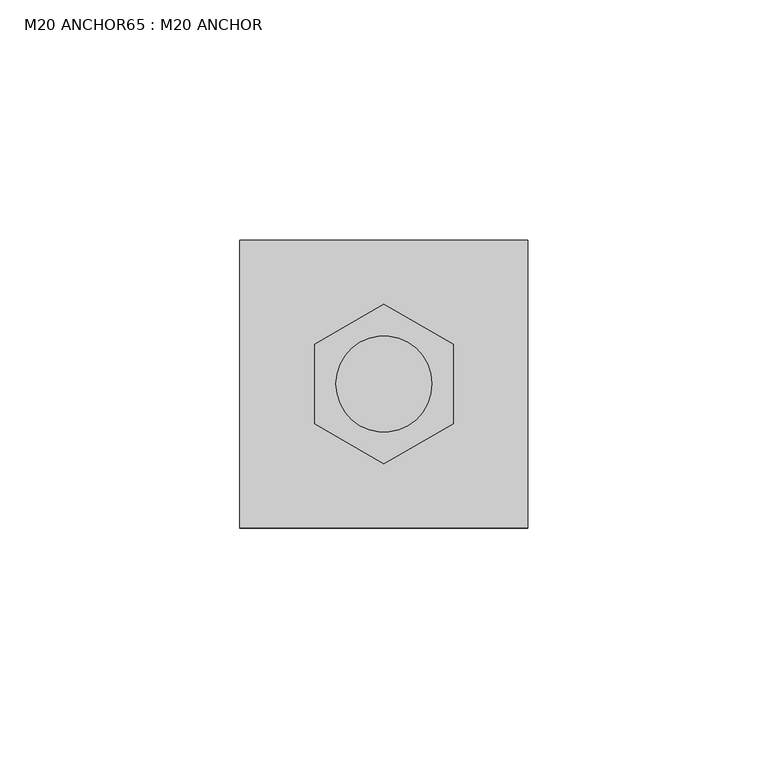
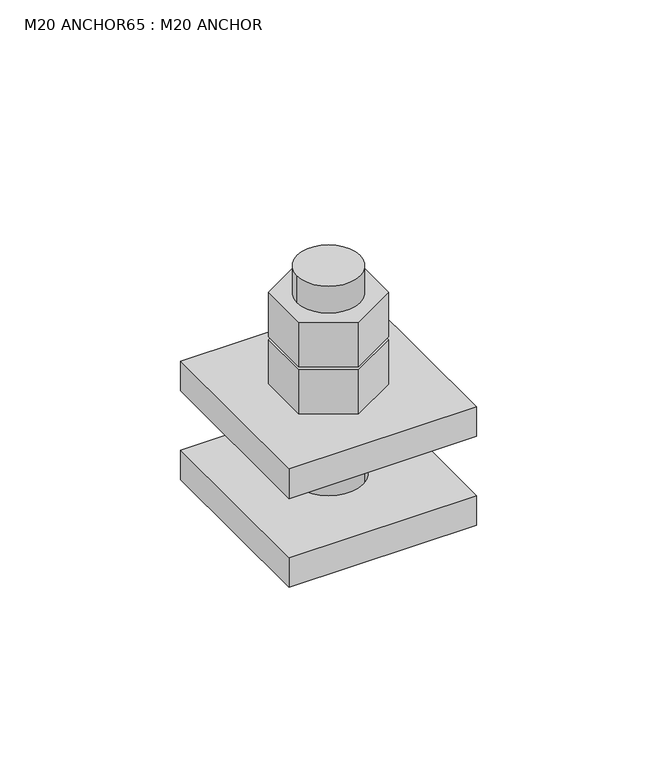
"""IFC4 building model written with IfcOpenShell, lengths in millimetres: fastener geometry, M20 ANCHOR65 : M20 ANCHOR."""

from ifc_helpers import new_model, si_unit, point, frame, frame_2d, origin, place, context, project, spatial, polyline, circle_curve, trimmed, segment, composite_curve, outline, extrude, source, transform, mapped, element, save


def m20_anchor65_m20_anchor_09f6851c(model_context):
    return source(origin(), model_context, "Body", "SweptSolid", [
        extrude(outline(polyline([(15008.0855968, 19453.9464399), (15008.0855968, 19470.5835027), (15022.4937158, 19478.9020341), (15036.9018348, 19470.5835027), (15036.9018348, 19453.9464399), (15022.4937158, 19445.6279085), (15008.0855968, 19453.9464399)]), holes=[composite_curve([segment(trimmed(circle_curve(frame_2d((15022.4937158, 19462.2649713)), 10.0), [point((15032.4937158, 19462.2649713))], [point((15012.4937158, 19462.2649713))], True, "CARTESIAN"), True, "CONTINUOUS"), segment(trimmed(circle_curve(frame_2d((15022.4937158, 19462.2649713)), 10.0), [point((15012.4937158, 19462.2649713))], [point((15032.4937158, 19462.2649713))], True, "CARTESIAN"), True, "CONTINUOUS")], self_intersect=False)]), frame((0.0, 0.0, 246.0), z_axis=(0.0, 0.0, 1.0), x_axis=(1.0, 0.0, 0.0)), (0.0, 0.0, 1.0), 15.0),
        extrude(outline(polyline([(15008.0855968, 19453.9464399), (15008.0855968, 19470.5835027), (15022.4937158, 19478.9020341), (15036.9018348, 19470.5835027), (15036.9018348, 19453.9464399), (15022.4937158, 19445.6279085), (15008.0855968, 19453.9464399)]), holes=[composite_curve([segment(trimmed(circle_curve(frame_2d((15022.4937158, 19462.2649713)), 10.0), [point((15032.4937158, 19462.2649713))], [point((15012.4937158, 19462.2649713))], True, "CARTESIAN"), True, "CONTINUOUS"), segment(trimmed(circle_curve(frame_2d((15022.4937158, 19462.2649713)), 10.0), [point((15012.4937158, 19462.2649713))], [point((15032.4937158, 19462.2649713))], True, "CARTESIAN"), True, "CONTINUOUS")], self_intersect=False)]), frame((0.0, 0.0, 230.0), z_axis=(0.0, 0.0, 1.0), x_axis=(1.0, 0.0, 0.0)), (0.0, 0.0, 1.0), 15.0),
        extrude(outline(composite_curve([segment(trimmed(circle_curve(frame_2d((15022.4937158, 19462.2649713)), 10.0), [point((15032.4937158, 19462.2649713))], [point((15012.4937158, 19462.2649713))], False, "CARTESIAN"), True, "CONTINUOUS"), segment(trimmed(circle_curve(frame_2d((15022.4937158, 19462.2649713)), 10.0), [point((15012.4937158, 19462.2649713))], [point((15032.4937158, 19462.2649713))], False, "CARTESIAN"), True, "CONTINUOUS")], self_intersect=False)), frame((0.0, 0.0, 190.0), z_axis=(0.0, 0.0, 1.0), x_axis=(1.0, 0.0, 0.0)), (0.0, 0.0, 1.0), 80.0),
        extrude(outline(polyline([(14992.4937158, 19432.2649713), (14992.4937158, 19492.2649713), (15052.4937158, 19492.2649713), (15052.4937158, 19432.2649713), (14992.4937158, 19432.2649713)]), holes=[composite_curve([segment(trimmed(circle_curve(frame_2d((15022.4937158, 19462.2649713)), 11.0), [point((15033.4937158, 19462.2649713))], [point((15011.4937158, 19462.2649713))], True, "CARTESIAN"), True, "CONTINUOUS"), segment(trimmed(circle_curve(frame_2d((15022.4937158, 19462.2649713)), 11.0), [point((15011.4937158, 19462.2649713))], [point((15033.4937158, 19462.2649713))], True, "CARTESIAN"), True, "CONTINUOUS")], self_intersect=False)]), frame((0.0, 0.0, 190.0), z_axis=(0.0, 0.0, 1.0), x_axis=(1.0, 0.0, 0.0)), (0.0, 0.0, 1.0), 10.0),
        extrude(outline(polyline([(14992.4937158, 19432.2649713), (14992.4937158, 19492.2649713), (15052.4937158, 19492.2649713), (15052.4937158, 19432.2649713), (14992.4937158, 19432.2649713)]), holes=[composite_curve([segment(trimmed(circle_curve(frame_2d((15022.4937158, 19462.2649713)), 11.0), [point((15033.4937158, 19462.2649713))], [point((15011.4937158, 19462.2649713))], True, "CARTESIAN"), True, "CONTINUOUS"), segment(trimmed(circle_curve(frame_2d((15022.4937158, 19462.2649713)), 11.0), [point((15011.4937158, 19462.2649713))], [point((15033.4937158, 19462.2649713))], True, "CARTESIAN"), True, "CONTINUOUS")], self_intersect=False)]), frame((0.0, 0.0, 220.0), z_axis=(0.0, 0.0, 1.0), x_axis=(1.0, 0.0, 0.0)), (0.0, 0.0, 1.0), 10.0),
    ])


if __name__ == "__main__":
    model = new_model("IFC4")
    model_context = context("Model", 3, world=origin())
    ifc_project = project(units=[si_unit("LENGTHUNIT", "METRE", prefix="MILLI")], contexts=[model_context])
    site = spatial("IfcSite", under=ifc_project)
    building = spatial("IfcBuilding", under=site)
    placement = place(None, origin())
    m20_anchor65_m20_anchor_shape = m20_anchor65_m20_anchor_09f6851c(model_context)
    element("IfcFastener", 1, ObjectType="M20 ANCHOR65 : M20 ANCHOR", at=placement, inside=building, context=model_context, shape_type="MappedRepresentation", body=[
        mapped(m20_anchor65_m20_anchor_shape, transform((0.0, 0.0, 0.0), x_axis=(1.0, 0.0, 0.0), y_axis=(0.0, 1.0, 0.0), z_axis=(0.0, 0.0, 1.0))),
    ])
    save(model, "model.ifc")
